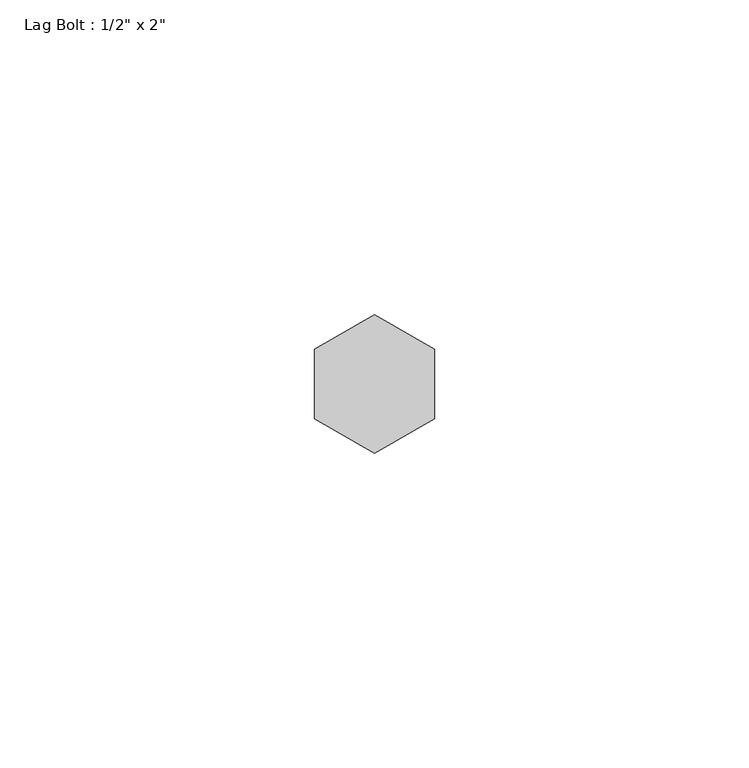
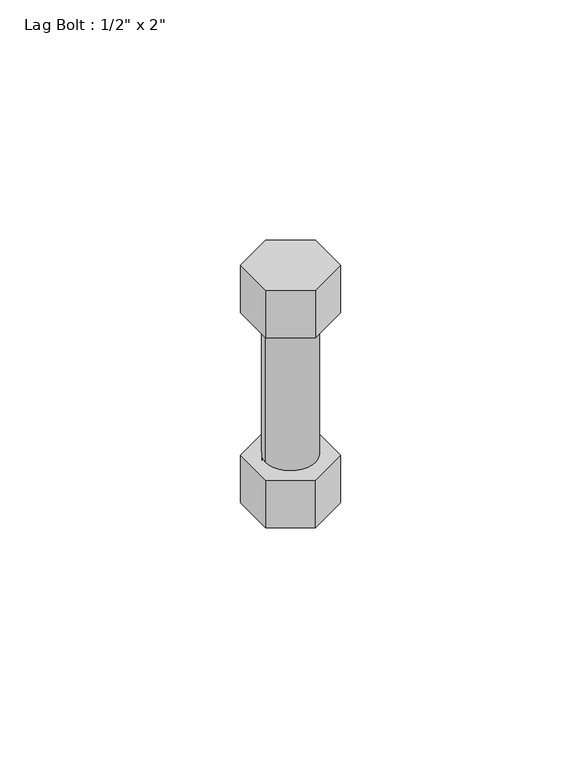
"""IFC4 building model written with IfcOpenShell, lengths in millimetres: proxy geometry."""

from ifc_helpers import new_model, si_unit, point, frame, origin, origin_with_axes, origin_2d, place, context, project, spatial, polyline, circle_curve, trimmed, segment, composite_curve, outline, extrude, source, transform, mapped, element, save


def proxy_66e8b3a5(model_context):
    return source(origin(), model_context, "Body", "SweptSolid", [
        extrude(outline(polyline([(-9.525, -5.4992613), (-9.525, 5.4992613), (0.0, 10.9985226), (9.525, 5.4992613), (9.525, -5.4992613), (0.0, -10.9985226), (-9.525, -5.4992613)])), frame((0.0, 0.0, -50.8), z_axis=(0.0, 0.0, 1.0), x_axis=(1.0, 0.0, 0.0)), (0.0, 0.0, 1.0), 12.7),
        extrude(outline(polyline([(-9.525, 5.4992613), (0.0, 10.9985226), (9.525, 5.4992613), (9.525, -5.4992613), (0.0, -10.9985226), (-9.525, -5.4992613), (-9.525, 5.4992613)])), origin_with_axes(), (0.0, 0.0, 1.0), 12.7),
        extrude(outline(composite_curve([segment(trimmed(circle_curve(origin_2d(), 6.35), [point((-6.35, 0.0))], [point((6.35, 0.0))], False, "CARTESIAN"), True, "CONTINUOUS"), segment(trimmed(circle_curve(origin_2d(), 6.35), [point((6.35, 0.0))], [point((-6.35, 0.0))], False, "CARTESIAN"), True, "CONTINUOUS")], self_intersect=False)), frame((0.0, 0.0, -50.8), z_axis=(0.0, 0.0, 1.0), x_axis=(1.0, 0.0, 0.0)), (0.0, 0.0, 1.0), 50.8),
    ])


if __name__ == "__main__":
    model = new_model("IFC4")
    model_context = context("Model", 3, world=origin())
    ifc_project = project(units=[si_unit("LENGTHUNIT", "METRE", prefix="MILLI")], contexts=[model_context])
    site = spatial("IfcSite", under=ifc_project)
    building = spatial("IfcBuilding", under=site)
    placement = place(None, origin())
    proxy_shape = proxy_66e8b3a5(model_context)
    element("IfcBuildingElementProxy", 1, Name="Lag Bolt : 1/2\" x 2\"", ObjectType="Lag Bolt : 1/2\" x 2\"", at=placement, inside=building, context=model_context, shape_type="MappedRepresentation", body=[
        mapped(proxy_shape, transform((0.0, 0.0, 0.0), x_axis=(1.0, 0.0, 0.0), y_axis=(0.0, 1.0, 0.0), z_axis=(0.0, 0.0, 1.0))),
    ])
    save(model, "model.ifc")

# Revit data of these elements
# Type "Lag Bolt : 1/2\" x 2\""
#   Thickness_of_Substrate [instance default] = 0' - 1"
#   Side = 0' - 0 111/256"
#   Radius = 0' - 0 1/4"
#   Length = 0' - 2"
#   Head Size = 0' - 0 3/4"
#   Head Radius = 0' - 0 3/8"
#   Head Height = 0' - 0 1/2"
#   Diameter = 0' - 0 1/2"
#   Default Elevation = 4' - 0"
#   Nut_Visibility [instance default] = yes
#   Bolt Material (Size) [instance default] = 1" GALV. LAG BOLT (LENGTH = 1/2" SHY OF GLULAM DEPTH) -  (GALV. THRU BOLT IF PLATE ON OPP. SIDE OF STRUCT MEMBER)
# Element 1 (IfcBuildingElementProxy, "Lag Bolt : 1/2\" x 2\"")
#   Thickness_of_Substrate = 0' - 1 1/2"
#   Bolt Material (Size) = 1/2 LAG BOLTS 24" O.C.
#   Materials on its faces: "1/2 LAG BOLTS 24\" O.C.", "STRUCTURAL BOLTS (PAINT TO MATCH STEEL FINISH)"
# Materials
#   "1\" GALV. LAG BOLT (LENGTH = 1/2\" SHY OF GLULAM DEPTH) -  (GALV. THRU BOLT IF PLATE ON OPP. SIDE OF STRUCT MEMBER)": class "Generic", colour RGB 120 120 120, transparency 0, Cost = 0
#   "1/2 LAG BOLTS 24\" O.C.": class "Generic", colour RGB 120 120 120, transparency 0, Cost = 0
#   "STRUCTURAL BOLTS (PAINT TO MATCH STEEL FINISH)": class "Generic", colour RGB 120 120 120, transparency 0, Cost = 0
